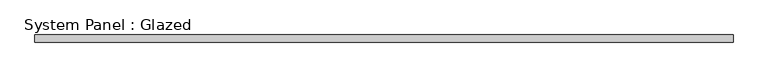
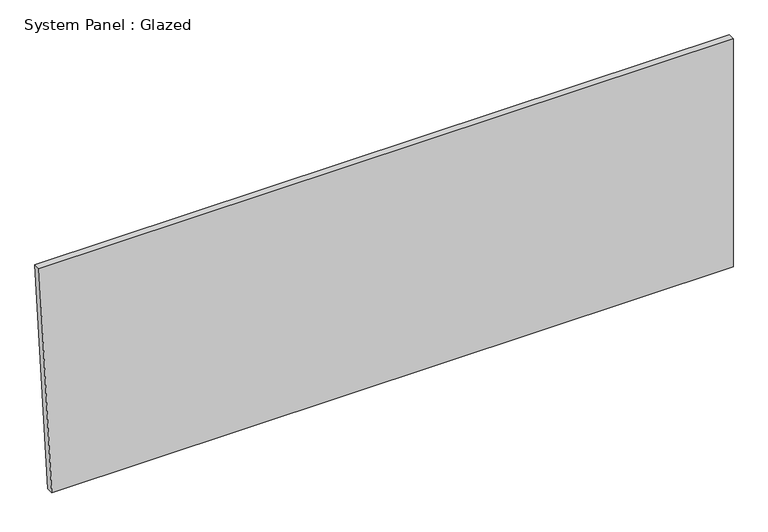
"""IFC4 building model written with IfcOpenShell, lengths in millimetres: plate geometry, System Panel : Glazed."""

from ifc_helpers import new_model, si_unit, frame, origin, place, context, project, spatial, polyline, outline, extrude, source, transform, mapped, element, save


def system_panel_glazed_1dbcaf42(model_context):
    return source(origin(), model_context, "Body", "SweptSolid", [
        extrude(outline(polyline([(0.0, -1202.0248119), (0.0, 1247.3520184), (866.081558, 1247.3520184), (866.081558, -1247.3520184), (0.0, -1202.0248119)])), frame((0.0, -44.45, 0.0), z_axis=(0.0, 1.0, 0.0), x_axis=(0.0, 0.0, 1.0)), (0.0, 0.0, 1.0), 25.4),
    ])


if __name__ == "__main__":
    model = new_model("IFC4")
    model_context = context("Model", 3, world=origin())
    ifc_project = project(units=[si_unit("LENGTHUNIT", "METRE", prefix="MILLI")], contexts=[model_context])
    site = spatial("IfcSite", under=ifc_project)
    building = spatial("IfcBuilding", under=site)
    placement = place(None, origin())
    system_panel_glazed_shape = system_panel_glazed_1dbcaf42(model_context)
    element("IfcPlate", 1, ObjectType="System Panel : Glazed", at=placement, inside=building, context=model_context, shape_type="MappedRepresentation", body=[
        mapped(system_panel_glazed_shape, transform((0.0, 0.0, 0.0), x_axis=(1.0, 0.0, 0.0), y_axis=(0.0, 1.0, 0.0), z_axis=(0.0, 0.0, 1.0))),
    ])
    save(model, "model.ifc")

# Revit data of these elements
# Type "System Panel : Glazed"
#   Construction Type Id = "GSP4R"
#   Analytic Construction = "1/8 in Pilkington single glazing"
#   Visual Light Transmittance = 0.9
#   Solar Heat Gain Coefficient = 0.86
#   Heat Transfer Coefficient (U) = 1.18115 BTU/(h·ft²·°F)
#   Define Thermal Properties by = 1
# Element 1 (IfcPlate, "System Panel : Glazed")
#   Materials on its faces: "Glass"
# Materials
#   "Glass": class "Glass", colour RGB 0 128 192, transparency 0.75, Description = "Soda Lime Glass", Cost = 0
